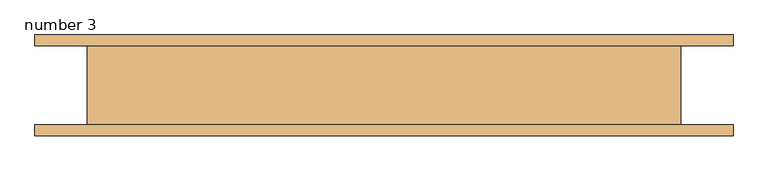
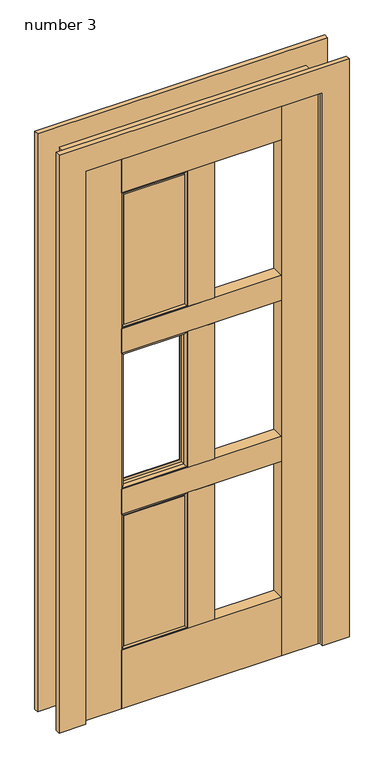
"""IFC4 building model written with IfcOpenShell, lengths in millimetres: door geometry, Door-Interior-Karona-K5660-6_Panel : number 3."""

from ifc_helpers import new_model, si_unit, frame, origin, origin_with_axes, place, context, project, spatial, polyline, ellipse_curve, outline, extrude, faceted_brep, source, transform, mapped, element, save
from ifc_brep_helpers import plane_surface, cylinder_surface, revolved_surface, advanced_brep


def number_3_9a47f452(model_context):
    return source(origin(), model_context, "Body", "SolidModel", [
        advanced_brep(
        [(-279.4, -15.2908, 1311.275), (-46.0375, -15.2908, 1311.275), (-57.3628137, -24.6126, 1299.9496863), (-268.0746863, -24.6126, 1299.9496863), (-57.1627, -46.3324899, 1300.1498), (-57.1627, -46.3324899, 820.7502), (-48.2727, -54.4576, 811.8602), (-48.2727, -54.4576, 1309.0398), (-268.2748, -46.3324899, 820.7502), (-268.2748, -46.3324899, 1300.1498), (-277.1648, -54.4576, 1309.0398), (-277.1648, -54.4576, 811.8602), (-46.0375, -54.4576, 809.625), (-279.4, -54.4576, 809.625), (-279.4, -15.2908, 809.625), (-46.0375, -15.2908, 809.625), (-57.1627, -34.7218, 820.7502), (-268.2748, -34.7218, 820.7502), (-47.3075, -24.6126, 1310.005), (-47.3075, -24.6126, 810.895), (-47.3075, -34.7218, 810.895), (-47.3075, -34.7218, 1310.005), (-278.13, -24.6126, 810.895), (-278.13, -24.6126, 1310.005), (-57.3628137, -24.6126, 820.9503137), (-268.0746863, -24.6126, 820.9503137), (-278.13, -34.7218, 810.895), (-279.4, -54.4576, 1311.275), (-268.2748, -34.7218, 1300.1498), (-278.13, -34.7218, 1310.005), (-46.0375, -54.4576, 1311.275), (-57.1627, -34.7218, 1300.1498)],
        [
            (0, 1),
            (1, 2, ellipse_curve(frame((-47.0685124, -25.5788135, 1310.2439876), z_axis=(-0.7071067811865475, 0.0, 0.7071067811865475), x_axis=(-0.7071067811865476, 0.0, -0.7071067811865474)), 14.6223259, 10.3395458)),
            (2, 3),
            (3, 0, ellipse_curve(frame((-278.3689876, -25.5788135, 1310.2439876), z_axis=(0.7071067811865475, 0.0, 0.7071067811865475), x_axis=(-0.7071067811865476, 0.0, 0.7071067811865474)), 14.6223259, 10.3395458)),
            (4, 5),
            (5, 6, ellipse_curve(frame((-48.2727, -45.531597, 811.8602), z_axis=(0.7071067811865475, 0.0, 0.7071067811865475), x_axis=(-0.7071067811865474, 0.0, 0.7071067811865476)), 12.6232745, 8.926003)),
            (6, 7),
            (7, 4, ellipse_curve(frame((-48.2727, -45.531597, 1309.0398), z_axis=(0.7071067811865475, 0.0, -0.7071067811865475), x_axis=(0.7071067811865474, 0.0, 0.7071067811865476)), 12.6232745, 8.926003)),
            (8, 9),
            (9, 10, ellipse_curve(frame((-277.1648, -45.531597, 1309.0398), z_axis=(-0.7071067811865475, 0.0, -0.7071067811865475), x_axis=(0.7071067811865474, 0.0, -0.7071067811865476)), 12.6232745, 8.926003)),
            (10, 11),
            (11, 8, ellipse_curve(frame((-277.1648, -45.531597, 811.8602), z_axis=(-0.7071067811865475, 0.0, 0.7071067811865475), x_axis=(-0.7071067811865474, 0.0, -0.7071067811865476)), 12.6232745, 8.926003)),
            (12, 13),
            (13, 14),
            (14, 15),
            (15, 12),
            (16, 17),
            (17, 8),
            (8, 5),
            (5, 16),
            (18, 19),
            (19, 20),
            (20, 21),
            (21, 18),
            (22, 19),
            (18, 23),
            (23, 22),
            (24, 25),
            (25, 3),
            (2, 24),
            (14, 25, ellipse_curve(frame((-278.3689876, -25.5788135, 810.6560124), z_axis=(0.7071067811865475, 0.0, -0.7071067811865475), x_axis=(0.7071067811865476, 0.0, 0.7071067811865474)), 14.6223259, 10.3395458)),
            (24, 15, ellipse_curve(frame((-47.0685124, -25.5788135, 810.6560124), z_axis=(-0.7071067811865475, 0.0, -0.7071067811865475), x_axis=(0.7071067811865476, 0.0, -0.7071067811865474)), 14.6223259, 10.3395458)),
            (22, 26),
            (26, 20),
            (13, 27),
            (27, 0),
            (0, 14),
            (17, 28),
            (28, 9),
            (23, 29),
            (29, 26),
            (27, 30),
            (30, 1),
            (28, 31),
            (31, 4),
            (4, 9),
            (21, 29),
            (30, 12),
            (15, 1),
            (31, 16),
            (6, 11),
            (10, 7),
        ],
        [
            cylinder_surface(frame((-279.4, -25.5788135, 1310.2439876), z_axis=(-1.0, 0.0, 0.0), x_axis=(0.0, 1.0, 0.0)), 10.3395458),
            cylinder_surface(frame((-48.2727, -45.531597, 1311.275), z_axis=(0.0, 0.0, 1.0), x_axis=(0.0, 1.0, 0.0)), 8.926003),
            cylinder_surface(frame((-277.1648, -45.531597, 809.625), z_axis=(0.0, 0.0, -1.0), x_axis=(0.0, 1.0, 0.0)), 8.926003),
            plane_surface(frame((-46.0375, -15.2908, 809.625), z_axis=(0.0, 0.0, -1.0), x_axis=(-1.0, 0.0, 0.0))),
            plane_surface(frame((-57.1627, -46.3324899, 820.7502), z_axis=(0.0, 0.0, 1.0), x_axis=(-1.0, 0.0, 0.0))),
            plane_surface(frame((-47.3075, -34.7218, 1310.005), z_axis=(-1.0, 0.0, 0.0), x_axis=(0.0, 0.0, -1.0))),
            plane_surface(frame((-47.3075, -24.6126, 1310.005), z_axis=(0.0, -1.0, 0.0), x_axis=(0.0, 0.0, -1.0))),
            cylinder_surface(frame((-46.0375, -25.5788135, 810.6560124), z_axis=(1.0, 0.0, 0.0), x_axis=(0.0, 1.0, 0.0)), 10.3395458),
            plane_surface(frame((-47.3075, -34.7218, 810.895), z_axis=(0.0, 0.0, 1.0), x_axis=(-1.0, 0.0, 0.0))),
            plane_surface(frame((-279.4, -15.2908, 809.625), z_axis=(-1.0, 0.0, 0.0), x_axis=(0.0, 0.0, 1.0))),
            plane_surface(frame((-268.2748, -46.3324899, 820.7502), z_axis=(1.0, 0.0, 0.0), x_axis=(0.0, 0.0, 1.0))),
            plane_surface(frame((-278.13, -34.7218, 810.895), z_axis=(1.0, 0.0, 0.0), x_axis=(0.0, 0.0, 1.0))),
            plane_surface(frame((-279.4, -15.2908, 1311.275), z_axis=(0.0, 0.0, 1.0), x_axis=(1.0, 0.0, 0.0))),
            plane_surface(frame((-268.2748, -46.3324899, 1300.1498), z_axis=(0.0, 0.0, -1.0), x_axis=(1.0, 0.0, 0.0))),
            plane_surface(frame((-278.13, -34.7218, 1310.005), z_axis=(0.0, 0.0, -1.0), x_axis=(1.0, 0.0, 0.0))),
            plane_surface(frame((-46.0375, -15.2908, 1311.275), z_axis=(1.0, 0.0, 0.0), x_axis=(0.0, 0.0, -1.0))),
            plane_surface(frame((-57.1627, -46.3324899, 1300.1498), z_axis=(-1.0, 0.0, 0.0), x_axis=(0.0, 0.0, -1.0))),
            plane_surface(frame((-57.1627, -34.7218, 1300.1498), z_axis=(0.0, 1.0, 0.0), x_axis=(0.0, 0.0, -1.0))),
            plane_surface(frame((-46.0375, -54.4576, 1311.275), z_axis=(0.0, -1.0, 0.0), x_axis=(0.0, 0.0, -1.0))),
            cylinder_surface(frame((-46.0375, -45.531597, 811.8602), z_axis=(1.0, 0.0, 0.0), x_axis=(0.0, 1.0, 0.0)), 8.926003),
            cylinder_surface(frame((-278.3689876, -25.5788135, 809.625), z_axis=(0.0, 0.0, -1.0), x_axis=(0.0, 1.0, 0.0)), 10.3395458),
            cylinder_surface(frame((-279.4, -45.531597, 1309.0398), z_axis=(-1.0, 0.0, 0.0), x_axis=(0.0, 1.0, 0.0)), 8.926003),
            cylinder_surface(frame((-47.0685124, -25.5788135, 1311.275), z_axis=(0.0, 0.0, 1.0), x_axis=(0.0, 1.0, 0.0)), 10.3395458),
        ],
        [
            (0, [[1, 2, 3, 4]]),
            (1, [[5, 6, 7, 8]]),
            (2, [[9, 10, 11, 12]]),
            (3, [[13, 14, 15, 16]]),
            (4, [[17, 18, 19, 20]]),
            (5, [[21, 22, 23, 24]]),
            (6, [[25, -21, 26, 27], [28, 29, -3, 30]]),
            (7, [[-15, 31, -28, 32]]),
            (8, [[-25, 33, 34, -22]]),
            (9, [[35, 36, 37, -14]]),
            (10, [[38, 39, -9, -18]]),
            (11, [[-27, 40, 41, -33]]),
            (12, [[42, 43, -1, -36]]),
            (13, [[44, 45, 46, -39]]),
            (14, [[-26, -24, 47, -40]]),
            (15, [[48, -16, 49, -43]]),
            (16, [[50, -20, -5, -45]]),
            (17, [[-34, -41, -47, -23], [-17, -50, -44, -38]]),
            (18, [[-13, -48, -42, -35], [51, -11, 52, -7]]),
            (19, [[-19, -12, -51, -6]]),
            (20, [[-37, -4, -29, -31]]),
            (21, [[-46, -8, -52, -10]]),
            (22, [[-49, -32, -30, -2]]),
        ],
    ),
        advanced_brep(
        [(-268.2748, -54.4576, 1893.8748), (-268.2748, -54.4576, 1414.4752), (-57.1627, -54.4576, 1414.4752), (-57.1627, -54.4576, 1893.8748), (-268.2748, -34.7218, 1893.8748), (-268.2748, -36.0454899, 1893.8748), (-57.1627, -36.0454899, 1893.8748), (-57.1627, -34.7218, 1893.8748), (-57.1627, -44.5515929, 1893.8748), (-268.2748, -44.5515929, 1893.8748), (-57.1627, -34.7218, 1414.4752), (-57.1627, -36.0454899, 1414.4752), (-268.2748, -36.0454899, 1414.4752), (-268.2748, -34.7218, 1414.4752), (-268.2748, -44.5515929, 1414.4752), (-57.1627, -44.5515929, 1414.4752), (-87.1686653, -44.5515929, 1863.8688347), (-238.2688347, -44.5515929, 1863.8688347), (-87.1686653, -44.5515929, 1444.4811653), (-238.2688347, -44.5515929, 1444.4811653)],
        [
            (0, 1),
            (1, 2),
            (2, 3),
            (3, 0),
            (4, 5),
            (5, 6),
            (6, 7),
            (7, 4),
            (3, 8),
            (8, 9),
            (9, 0),
            (10, 11),
            (11, 12),
            (12, 13),
            (13, 10),
            (1, 14),
            (14, 15),
            (15, 2),
            (9, 14),
            (12, 5),
            (4, 13),
            (6, 11),
            (10, 7),
            (15, 8),
            (16, 6, ellipse_curve(frame((-55.2243315, -100.0605261, 1895.8131685), z_axis=(0.7071067811865475, 0.0, -0.7071067811865475), x_axis=(-0.7071067811865476, 0.0, -0.7071067811865474)), 90.5724254, 64.0443762)),
            (5, 17, ellipse_curve(frame((-270.2131685, -100.0605261, 1895.8131685), z_axis=(-0.7071067811865475, 0.0, -0.7071067811865475), x_axis=(-0.7071067811865476, 0.0, 0.7071067811865474)), 90.5724254, 64.0443762)),
            (17, 16),
            (18, 11, ellipse_curve(frame((-55.2243315, -100.0605261, 1412.5368315), z_axis=(-0.7071067811865475, 0.0, -0.7071067811865475), x_axis=(-0.7071067811865474, 0.0, 0.7071067811865476)), 90.5724254, 64.0443762)),
            (16, 18),
            (19, 12, ellipse_curve(frame((-270.2131685, -100.0605261, 1412.5368315), z_axis=(-0.7071067811865475, 0.0, 0.7071067811865475), x_axis=(0.7071067811865476, 0.0, 0.7071067811865474)), 90.5724254, 64.0443762)),
            (18, 19),
            (19, 17),
        ],
        [
            plane_surface(frame((-57.1627, -54.4576, 1893.8748), z_axis=(0.0, -1.0, 0.0), x_axis=(0.0, 0.0, -1.0))),
            plane_surface(frame((-57.1627, -34.7218, 1893.8748), z_axis=(0.0, 0.0, 1.0), x_axis=(1.0, 0.0, 0.0))),
            plane_surface(frame((-57.1627, -34.7218, 1414.4752), z_axis=(0.0, 0.0, -1.0), x_axis=(-1.0, 0.0, 0.0))),
            plane_surface(frame((-268.2748, -54.4576, 1893.8748), z_axis=(-1.0, 0.0, 0.0), x_axis=(0.0, 0.0, -1.0))),
            plane_surface(frame((-57.1627, -34.7218, 1893.8748), z_axis=(1.0, 0.0, 0.0), x_axis=(0.0, 0.0, -1.0))),
            plane_surface(frame((-268.2748, -34.7218, 1893.8748), z_axis=(0.0, 1.0, 0.0), x_axis=(0.0, 0.0, -1.0))),
            revolved_surface(polyline([(-334.2575446888527, -100.0605261, 1831.7687923), (8.820044688852704, -100.0605261, 1831.7687923)]), (-279.4, -100.0605261, 1895.8131685), (-1.0, 0.0, 0.0)),
            revolved_surface(polyline([(-119.2687077, -100.0605261, 1959.8575446888528), (-119.2687077, -100.0605261, 1348.4924553111473)]), (-55.2243315, -100.0605261, 1905.0), (0.0, 0.0, 1.0)),
            revolved_surface(polyline([(8.820044688852683, -100.0605261, 1476.5812077), (-334.2575446888527, -100.0605261, 1476.5812077)]), (-46.0375, -100.0605261, 1412.5368315), (1.0, 0.0, 0.0)),
            revolved_surface(polyline([(-206.1687923, -100.0605261, 1348.4924553111473), (-206.1687923, -100.0605261, 1959.8575446888526)]), (-270.2131685, -100.0605261, 1403.35), (0.0, 0.0, -1.0)),
            plane_surface(frame((-279.4, -44.5515929, 1403.35), z_axis=(0.0, 1.0, 0.0), x_axis=(0.0, 0.0, 1.0))),
        ],
        [
            (0, [[1, 2, 3, 4]]),
            (1, [[5, 6, 7, 8]]),
            (1, [[9, 10, 11, -4]]),
            (2, [[12, 13, 14, 15]]),
            (2, [[16, 17, 18, -2]]),
            (3, [[-11, 19, -16, -1]]),
            (3, [[-14, 20, -5, 21]]),
            (4, [[-7, 22, -12, 23]]),
            (4, [[-18, 24, -9, -3]]),
            (5, [[-23, -15, -21, -8]]),
            (6, [[25, -6, 26, 27]]),
            (7, [[28, -22, -25, 29]]),
            (8, [[30, -13, -28, 31]]),
            (9, [[-26, -20, -30, 32]]),
            (10, [[-24, -17, -19, -10], [-32, -31, -29, -27]]),
        ],
    ),
        advanced_brep(
        [(-268.2748, -24.6126, 1893.8748), (-268.2748, -24.6126, 1414.4752), (-57.1627, -24.6126, 1414.4752), (-57.1627, -24.6126, 1893.8748), (-239.4448579, -15.4432, 1443.3051421), (-239.4448579, -15.4432, 1865.0448579), (-85.9926421, -15.4432, 1865.0448579), (-85.9926421, -15.4432, 1443.3051421), (-57.1627, -23.2889101, 1893.8748), (-268.2748, -23.2889101, 1893.8748), (-268.2748, -23.2889101, 1414.4752), (-57.1627, -23.2889101, 1414.4752)],
        [
            (0, 1),
            (1, 2),
            (2, 3),
            (3, 0),
            (4, 5),
            (5, 6),
            (6, 7),
            (7, 4),
            (3, 8),
            (8, 9),
            (9, 0),
            (1, 10),
            (10, 11),
            (11, 2),
            (7, 11, ellipse_curve(frame((-55.2243315, 40.7261261, 1412.5368315), z_axis=(0.7071067811865475, 0.0, 0.7071067811865475), x_axis=(0.7071067811865476, 0.0, -0.7071067811865474)), 90.5724254, 64.0443762)),
            (10, 4, ellipse_curve(frame((-270.2131685, 40.7261261, 1412.5368315), z_axis=(-0.7071067811865475, 0.0, 0.7071067811865475), x_axis=(0.7071067811865476, 0.0, 0.7071067811865474)), 90.5724254, 64.0443762)),
            (10, 9),
            (9, 5, ellipse_curve(frame((-270.2131685, 40.7261261, 1895.8131685), z_axis=(0.7071067811865475, 0.0, 0.7071067811865475), x_axis=(0.7071067811865474, 0.0, -0.7071067811865476)), 90.5724254, 64.0443762)),
            (8, 6, ellipse_curve(frame((-55.2243315, 40.7261261, 1895.8131685), z_axis=(0.7071067811865475, 0.0, -0.7071067811865475), x_axis=(-0.7071067811865476, 0.0, -0.7071067811865474)), 90.5724254, 64.0443762)),
            (8, 11),
        ],
        [
            plane_surface(frame((-57.1627, -24.6126, 1893.8748), z_axis=(0.0, -1.0, 0.0), x_axis=(0.0, 0.0, -1.0))),
            plane_surface(frame((-268.2748, -15.4432, 1893.8748), z_axis=(0.0, 1.0, 0.0), x_axis=(0.0, 0.0, -1.0))),
            plane_surface(frame((-57.1627, -34.7218, 1893.8748), z_axis=(0.0, 0.0, 1.0), x_axis=(1.0, 0.0, 0.0))),
            plane_surface(frame((-57.1627, -34.7218, 1414.4752), z_axis=(0.0, 0.0, -1.0), x_axis=(-1.0, 0.0, 0.0))),
            revolved_surface(polyline([(8.820044688852711, 40.7261261, 1476.5812077), (-334.2575446888527, 40.7261261, 1476.5812077)]), (-46.0375, 40.7261261, 1412.5368315), (1.0, 0.0, 0.0)),
            revolved_surface(polyline([(-206.1687923, 40.7261261, 1348.4924553111473), (-206.1687923, 40.7261261, 1959.8575446888528)]), (-270.2131685, 40.7261261, 1403.35), (0.0, 0.0, -1.0)),
            revolved_surface(polyline([(-334.2575446888527, 40.7261261, 1831.7687923), (8.820044688852704, 40.7261261, 1831.7687923)]), (-279.4, 40.7261261, 1895.8131685), (-1.0, 0.0, 0.0)),
            revolved_surface(polyline([(-119.2687077, 40.7261261, 1959.8575446888528), (-119.2687077, 40.7261261, 1348.4924553111473)]), (-55.2243315, 40.7261261, 1905.0), (0.0, 0.0, 1.0)),
            plane_surface(frame((-268.2748, -24.6126, 1893.8748), z_axis=(-1.0, 0.0, 0.0), x_axis=(0.0, 0.0, -1.0))),
            plane_surface(frame((-57.1627, -15.4432, 1893.8748), z_axis=(1.0, 0.0, 0.0), x_axis=(0.0, 0.0, -1.0))),
        ],
        [
            (0, [[1, 2, 3, 4]]),
            (1, [[5, 6, 7, 8]]),
            (2, [[9, 10, 11, -4]]),
            (3, [[12, 13, 14, -2]]),
            (4, [[-8, 15, -13, 16]]),
            (5, [[17, 18, -5, -16]]),
            (6, [[-10, 19, -6, -18]]),
            (7, [[20, -15, -7, -19]]),
            (8, [[-11, -17, -12, -1]]),
            (9, [[-14, -20, -9, -3]]),
        ],
    ),
        advanced_brep(
        [(-279.4, -15.2908, 1905.0), (-46.0375, -15.2908, 1905.0), (-57.3628137, -24.6126, 1893.6746863), (-268.0746863, -24.6126, 1893.6746863), (-57.1627, -46.3324899, 1893.8748), (-57.1627, -46.3324899, 1414.4752), (-48.2727, -54.4576, 1405.5852), (-48.2727, -54.4576, 1902.7648), (-268.2748, -46.3324899, 1414.4752), (-268.2748, -46.3324899, 1893.8748), (-277.1648, -54.4576, 1902.7648), (-277.1648, -54.4576, 1405.5852), (-46.0375, -54.4576, 1403.35), (-279.4, -54.4576, 1403.35), (-279.4, -15.2908, 1403.35), (-46.0375, -15.2908, 1403.35), (-57.1627, -34.7218, 1414.4752), (-268.2748, -34.7218, 1414.4752), (-47.3075, -24.6126, 1903.73), (-47.3075, -24.6126, 1404.62), (-47.3075, -34.7218, 1404.62), (-47.3075, -34.7218, 1903.73), (-278.13, -24.6126, 1404.62), (-278.13, -24.6126, 1903.73), (-57.3628137, -24.6126, 1414.6753137), (-268.0746863, -24.6126, 1414.6753137), (-278.13, -34.7218, 1404.62), (-279.4, -54.4576, 1905.0), (-268.2748, -34.7218, 1893.8748), (-278.13, -34.7218, 1903.73), (-46.0375, -54.4576, 1905.0), (-57.1627, -34.7218, 1893.8748)],
        [
            (0, 1),
            (1, 2, ellipse_curve(frame((-47.0685124, -25.5788135, 1903.9689876), z_axis=(-0.7071067811865475, 0.0, 0.7071067811865475), x_axis=(-0.7071067811865476, 0.0, -0.7071067811865474)), 14.6223259, 10.3395458)),
            (2, 3),
            (3, 0, ellipse_curve(frame((-278.3689876, -25.5788135, 1903.9689876), z_axis=(0.7071067811865475, 0.0, 0.7071067811865475), x_axis=(-0.7071067811865476, 0.0, 0.7071067811865474)), 14.6223259, 10.3395458)),
            (4, 5),
            (5, 6, ellipse_curve(frame((-48.2727, -45.531597, 1405.5852), z_axis=(0.7071067811865475, 0.0, 0.7071067811865475), x_axis=(-0.7071067811865474, 0.0, 0.7071067811865476)), 12.6232745, 8.926003)),
            (6, 7),
            (7, 4, ellipse_curve(frame((-48.2727, -45.531597, 1902.7648), z_axis=(0.7071067811865475, 0.0, -0.7071067811865475), x_axis=(0.7071067811865474, 0.0, 0.7071067811865476)), 12.6232745, 8.926003)),
            (8, 9),
            (9, 10, ellipse_curve(frame((-277.1648, -45.531597, 1902.7648), z_axis=(-0.7071067811865475, 0.0, -0.7071067811865475), x_axis=(0.7071067811865474, 0.0, -0.7071067811865476)), 12.6232745, 8.926003)),
            (10, 11),
            (11, 8, ellipse_curve(frame((-277.1648, -45.531597, 1405.5852), z_axis=(-0.7071067811865475, 0.0, 0.7071067811865475), x_axis=(-0.7071067811865474, 0.0, -0.7071067811865476)), 12.6232745, 8.926003)),
            (12, 13),
            (13, 14),
            (14, 15),
            (15, 12),
            (16, 17),
            (17, 8),
            (8, 5),
            (5, 16),
            (18, 19),
            (19, 20),
            (20, 21),
            (21, 18),
            (22, 19),
            (18, 23),
            (23, 22),
            (24, 25),
            (25, 3),
            (2, 24),
            (14, 25, ellipse_curve(frame((-278.3689876, -25.5788135, 1404.3810124), z_axis=(0.7071067811865475, 0.0, -0.7071067811865475), x_axis=(0.7071067811865476, 0.0, 0.7071067811865474)), 14.6223259, 10.3395458)),
            (24, 15, ellipse_curve(frame((-47.0685124, -25.5788135, 1404.3810124), z_axis=(-0.7071067811865475, 0.0, -0.7071067811865475), x_axis=(0.7071067811865476, 0.0, -0.7071067811865474)), 14.6223259, 10.3395458)),
            (22, 26),
            (26, 20),
            (13, 27),
            (27, 0),
            (0, 14),
            (17, 28),
            (28, 9),
            (23, 29),
            (29, 26),
            (27, 30),
            (30, 1),
            (28, 31),
            (31, 4),
            (4, 9),
            (21, 29),
            (30, 12),
            (15, 1),
            (31, 16),
            (6, 11),
            (10, 7),
        ],
        [
            cylinder_surface(frame((-279.4, -25.5788135, 1903.9689876), z_axis=(-1.0, 0.0, 0.0), x_axis=(0.0, 1.0, 0.0)), 10.3395458),
            cylinder_surface(frame((-48.2727, -45.531597, 1905.0), z_axis=(0.0, 0.0, 1.0), x_axis=(0.0, 1.0, 0.0)), 8.926003),
            cylinder_surface(frame((-277.1648, -45.531597, 1403.35), z_axis=(0.0, 0.0, -1.0), x_axis=(0.0, 1.0, 0.0)), 8.926003),
            plane_surface(frame((-46.0375, -15.2908, 1403.35), z_axis=(0.0, 0.0, -1.0), x_axis=(-1.0, 0.0, 0.0))),
            plane_surface(frame((-57.1627, -46.3324899, 1414.4752), z_axis=(0.0, 0.0, 1.0), x_axis=(-1.0, 0.0, 0.0))),
            plane_surface(frame((-47.3075, -34.7218, 1903.73), z_axis=(-1.0, 0.0, 0.0), x_axis=(0.0, 0.0, -1.0))),
            plane_surface(frame((-47.3075, -24.6126, 1903.73), z_axis=(0.0, -1.0, 0.0), x_axis=(0.0, 0.0, -1.0))),
            cylinder_surface(frame((-46.0375, -25.5788135, 1404.3810124), z_axis=(1.0, 0.0, 0.0), x_axis=(0.0, 1.0, 0.0)), 10.3395458),
            plane_surface(frame((-47.3075, -34.7218, 1404.62), z_axis=(0.0, 0.0, 1.0), x_axis=(-1.0, 0.0, 0.0))),
            plane_surface(frame((-279.4, -15.2908, 1403.35), z_axis=(-1.0, 0.0, 0.0), x_axis=(0.0, 0.0, 1.0))),
            plane_surface(frame((-268.2748, -46.3324899, 1414.4752), z_axis=(1.0, 0.0, 0.0), x_axis=(0.0, 0.0, 1.0))),
            plane_surface(frame((-278.13, -34.7218, 1404.62), z_axis=(1.0, 0.0, 0.0), x_axis=(0.0, 0.0, 1.0))),
            plane_surface(frame((-279.4, -15.2908, 1905.0), z_axis=(0.0, 0.0, 1.0), x_axis=(1.0, 0.0, 0.0))),
            plane_surface(frame((-268.2748, -46.3324899, 1893.8748), z_axis=(0.0, 0.0, -1.0), x_axis=(1.0, 0.0, 0.0))),
            plane_surface(frame((-278.13, -34.7218, 1903.73), z_axis=(0.0, 0.0, -1.0), x_axis=(1.0, 0.0, 0.0))),
            plane_surface(frame((-46.0375, -15.2908, 1905.0), z_axis=(1.0, 0.0, 0.0), x_axis=(0.0, 0.0, -1.0))),
            plane_surface(frame((-57.1627, -46.3324899, 1893.8748), z_axis=(-1.0, 0.0, 0.0), x_axis=(0.0, 0.0, -1.0))),
            plane_surface(frame((-57.1627, -34.7218, 1893.8748), z_axis=(0.0, 1.0, 0.0), x_axis=(0.0, 0.0, -1.0))),
            plane_surface(frame((-46.0375, -54.4576, 1905.0), z_axis=(0.0, -1.0, 0.0), x_axis=(0.0, 0.0, -1.0))),
            cylinder_surface(frame((-46.0375, -45.531597, 1405.5852), z_axis=(1.0, 0.0, 0.0), x_axis=(0.0, 1.0, 0.0)), 8.926003),
            cylinder_surface(frame((-278.3689876, -25.5788135, 1403.35), z_axis=(0.0, 0.0, -1.0), x_axis=(0.0, 1.0, 0.0)), 10.3395458),
            cylinder_surface(frame((-279.4, -45.531597, 1902.7648), z_axis=(-1.0, 0.0, 0.0), x_axis=(0.0, 1.0, 0.0)), 8.926003),
            cylinder_surface(frame((-47.0685124, -25.5788135, 1905.0), z_axis=(0.0, 0.0, 1.0), x_axis=(0.0, 1.0, 0.0)), 10.3395458),
        ],
        [
            (0, [[1, 2, 3, 4]]),
            (1, [[5, 6, 7, 8]]),
            (2, [[9, 10, 11, 12]]),
            (3, [[13, 14, 15, 16]]),
            (4, [[17, 18, 19, 20]]),
            (5, [[21, 22, 23, 24]]),
            (6, [[25, -21, 26, 27], [28, 29, -3, 30]]),
            (7, [[-15, 31, -28, 32]]),
            (8, [[-25, 33, 34, -22]]),
            (9, [[35, 36, 37, -14]]),
            (10, [[38, 39, -9, -18]]),
            (11, [[-27, 40, 41, -33]]),
            (12, [[42, 43, -1, -36]]),
            (13, [[44, 45, 46, -39]]),
            (14, [[-26, -24, 47, -40]]),
            (15, [[48, -16, 49, -43]]),
            (16, [[50, -20, -5, -45]]),
            (17, [[-34, -41, -47, -23], [-17, -50, -44, -38]]),
            (18, [[-13, -48, -42, -35], [51, -11, 52, -7]]),
            (19, [[-19, -12, -51, -6]]),
            (20, [[-37, -4, -29, -31]]),
            (21, [[-46, -8, -52, -10]]),
            (22, [[-49, -32, -30, -2]]),
        ],
    ),
        advanced_brep(
        [(-268.2748, -34.7218, 706.4248), (-268.2748, -36.0454899, 706.4248), (-57.1627, -36.0454899, 706.4248), (-57.1627, -34.7218, 706.4248), (-57.1627, -54.4576, 706.4248), (-57.1627, -44.5515929, 706.4248), (-268.2748, -44.5515929, 706.4248), (-268.2748, -54.4576, 706.4248), (-57.1627, -34.7218, 227.0252), (-57.1627, -36.0454899, 227.0252), (-268.2748, -36.0454899, 227.0252), (-268.2748, -34.7218, 227.0252), (-268.2748, -54.4576, 227.0252), (-268.2748, -44.5515929, 227.0252), (-57.1627, -44.5515929, 227.0252), (-57.1627, -54.4576, 227.0252), (-87.1686653, -44.5515929, 676.4188347), (-238.2688347, -44.5515929, 676.4188347), (-87.1686653, -44.5515929, 257.0311653), (-238.2688347, -44.5515929, 257.0311653)],
        [
            (0, 1),
            (1, 2),
            (2, 3),
            (3, 0),
            (4, 5),
            (5, 6),
            (6, 7),
            (7, 4),
            (8, 9),
            (9, 10),
            (10, 11),
            (11, 8),
            (12, 13),
            (13, 14),
            (14, 15),
            (15, 12),
            (6, 13),
            (12, 7),
            (10, 1),
            (0, 11),
            (15, 4),
            (2, 9),
            (8, 3),
            (14, 5),
            (16, 2, ellipse_curve(frame((-55.2243315, -100.0605261, 708.3631685), z_axis=(0.7071067811865475, 0.0, -0.7071067811865475), x_axis=(-0.7071067811865476, 0.0, -0.7071067811865474)), 90.5724254, 64.0443762)),
            (1, 17, ellipse_curve(frame((-270.2131685, -100.0605261, 708.3631685), z_axis=(-0.7071067811865475, 0.0, -0.7071067811865475), x_axis=(-0.7071067811865476, 0.0, 0.7071067811865474)), 90.5724254, 64.0443762)),
            (17, 16),
            (18, 9, ellipse_curve(frame((-55.2243315, -100.0605261, 225.0868315), z_axis=(-0.7071067811865475, 0.0, -0.7071067811865475), x_axis=(-0.7071067811865474, 0.0, 0.7071067811865476)), 90.5724254, 64.0443762)),
            (16, 18),
            (19, 10, ellipse_curve(frame((-270.2131685, -100.0605261, 225.0868315), z_axis=(-0.7071067811865475, 0.0, 0.7071067811865475), x_axis=(0.7071067811865476, 0.0, 0.7071067811865474)), 90.5724254, 64.0443762)),
            (18, 19),
            (19, 17),
        ],
        [
            plane_surface(frame((-57.1627, -34.7218, 706.4248), z_axis=(0.0, 0.0, 1.0), x_axis=(1.0, 0.0, 0.0))),
            plane_surface(frame((-57.1627, -34.7218, 227.0252), z_axis=(0.0, 0.0, -1.0), x_axis=(-1.0, 0.0, 0.0))),
            plane_surface(frame((-268.2748, -54.4576, 706.4248), z_axis=(-1.0, 0.0, 0.0), x_axis=(0.0, 0.0, -1.0))),
            plane_surface(frame((-57.1627, -54.4576, 706.4248), z_axis=(0.0, -1.0, 0.0), x_axis=(0.0, 0.0, -1.0))),
            plane_surface(frame((-57.1627, -34.7218, 706.4248), z_axis=(1.0, 0.0, 0.0), x_axis=(0.0, 0.0, -1.0))),
            plane_surface(frame((-268.2748, -34.7218, 706.4248), z_axis=(0.0, 1.0, 0.0), x_axis=(0.0, 0.0, -1.0))),
            revolved_surface(polyline([(-334.2575446888527, -100.0605261, 644.3187923), (8.820044688852704, -100.0605261, 644.3187923)]), (-279.4, -100.0605261, 708.3631685), (-1.0, 0.0, 0.0)),
            revolved_surface(polyline([(-119.2687077, -100.0605261, 772.4075446888527), (-119.2687077, -100.0605261, 161.04245531114725)]), (-55.2243315, -100.0605261, 717.55), (0.0, 0.0, 1.0)),
            revolved_surface(polyline([(8.820044688852683, -100.0605261, 289.1312077), (-334.2575446888527, -100.0605261, 289.1312077)]), (-46.0375, -100.0605261, 225.0868315), (1.0, 0.0, 0.0)),
            revolved_surface(polyline([(-206.1687923, -100.0605261, 161.0424553111473), (-206.1687923, -100.0605261, 772.4075446888527)]), (-270.2131685, -100.0605261, 215.9), (0.0, 0.0, -1.0)),
            plane_surface(frame((-279.4, -44.5515929, 215.9), z_axis=(0.0, 1.0, 0.0), x_axis=(0.0, 0.0, 1.0))),
        ],
        [
            (0, [[1, 2, 3, 4]]),
            (0, [[5, 6, 7, 8]]),
            (1, [[9, 10, 11, 12]]),
            (1, [[13, 14, 15, 16]]),
            (2, [[-7, 17, -13, 18]]),
            (2, [[-11, 19, -1, 20]]),
            (3, [[-18, -16, 21, -8]]),
            (4, [[-3, 22, -9, 23]]),
            (4, [[-15, 24, -5, -21]]),
            (5, [[-23, -12, -20, -4]]),
            (6, [[25, -2, 26, 27]]),
            (7, [[28, -22, -25, 29]]),
            (8, [[30, -10, -28, 31]]),
            (9, [[-26, -19, -30, 32]]),
            (10, [[-24, -14, -17, -6], [-32, -31, -29, -27]]),
        ],
    ),
        advanced_brep(
        [(-57.1627, -24.6126, 706.4248), (-57.1627, -23.2889101, 706.4248), (-268.2748, -23.2889101, 706.4248), (-268.2748, -24.6126, 706.4248), (-268.2748, -24.6126, 227.0252), (-268.2748, -23.2889101, 227.0252), (-57.1627, -23.2889101, 227.0252), (-57.1627, -24.6126, 227.0252), (-239.4448579, -15.4432, 255.8551421), (-239.4448579, -15.4432, 677.5948579), (-85.9926421, -15.4432, 677.5948579), (-85.9926421, -15.4432, 255.8551421)],
        [
            (0, 1),
            (1, 2),
            (2, 3),
            (3, 0),
            (4, 5),
            (5, 6),
            (6, 7),
            (7, 4),
            (3, 4),
            (7, 0),
            (8, 9),
            (9, 10),
            (10, 11),
            (11, 8),
            (11, 6, ellipse_curve(frame((-55.2243315, 40.7261261, 225.0868315), z_axis=(0.7071067811865475, 0.0, 0.7071067811865475), x_axis=(0.7071067811865476, 0.0, -0.7071067811865474)), 90.5724254, 64.0443762)),
            (5, 8, ellipse_curve(frame((-270.2131685, 40.7261261, 225.0868315), z_axis=(-0.7071067811865475, 0.0, 0.7071067811865475), x_axis=(0.7071067811865476, 0.0, 0.7071067811865474)), 90.5724254, 64.0443762)),
            (5, 2),
            (2, 9, ellipse_curve(frame((-270.2131685, 40.7261261, 708.3631685), z_axis=(0.7071067811865475, 0.0, 0.7071067811865475), x_axis=(0.7071067811865474, 0.0, -0.7071067811865476)), 90.5724254, 64.0443762)),
            (1, 10, ellipse_curve(frame((-55.2243315, 40.7261261, 708.3631685), z_axis=(0.7071067811865475, 0.0, -0.7071067811865475), x_axis=(-0.7071067811865476, 0.0, -0.7071067811865474)), 90.5724254, 64.0443762)),
            (1, 6),
        ],
        [
            plane_surface(frame((-57.1627, -34.7218, 706.4248), z_axis=(0.0, 0.0, 1.0), x_axis=(1.0, 0.0, 0.0))),
            plane_surface(frame((-57.1627, -34.7218, 227.0252), z_axis=(0.0, 0.0, -1.0), x_axis=(-1.0, 0.0, 0.0))),
            plane_surface(frame((-57.1627, -24.6126, 706.4248), z_axis=(0.0, -1.0, 0.0), x_axis=(0.0, 0.0, -1.0))),
            plane_surface(frame((-268.2748, -15.4432, 706.4248), z_axis=(0.0, 1.0, 0.0), x_axis=(0.0, 0.0, -1.0))),
            revolved_surface(polyline([(8.820044688852711, 40.7261261, 289.1312077), (-334.2575446888527, 40.7261261, 289.1312077)]), (-46.0375, 40.7261261, 225.0868315), (1.0, 0.0, 0.0)),
            revolved_surface(polyline([(-206.1687923, 40.7261261, 161.0424553111473), (-206.1687923, 40.7261261, 772.4075446888527)]), (-270.2131685, 40.7261261, 215.9), (0.0, 0.0, -1.0)),
            revolved_surface(polyline([(-334.2575446888527, 40.7261261, 644.3187923), (8.820044688852704, 40.7261261, 644.3187923)]), (-279.4, 40.7261261, 708.3631685), (-1.0, 0.0, 0.0)),
            revolved_surface(polyline([(-119.2687077, 40.7261261, 772.4075446888527), (-119.2687077, 40.7261261, 161.04245531114736)]), (-55.2243315, 40.7261261, 717.55), (0.0, 0.0, 1.0)),
            plane_surface(frame((-268.2748, -24.6126, 706.4248), z_axis=(-1.0, 0.0, 0.0), x_axis=(0.0, 0.0, -1.0))),
            plane_surface(frame((-57.1627, -15.4432, 706.4248), z_axis=(1.0, 0.0, 0.0), x_axis=(0.0, 0.0, -1.0))),
        ],
        [
            (0, [[1, 2, 3, 4]]),
            (1, [[5, 6, 7, 8]]),
            (2, [[9, -8, 10, -4]]),
            (3, [[11, 12, 13, 14]]),
            (4, [[-14, 15, -6, 16]]),
            (5, [[17, 18, -11, -16]]),
            (6, [[-2, 19, -12, -18]]),
            (7, [[20, -15, -13, -19]]),
            (8, [[-3, -17, -5, -9]]),
            (9, [[-7, -20, -1, -10]]),
        ],
    ),
        advanced_brep(
        [(-279.4, -15.2908, 717.55), (-46.0375, -15.2908, 717.55), (-57.3628137, -24.6126, 706.2246863), (-268.0746863, -24.6126, 706.2246863), (-57.1627, -46.3324899, 706.4248), (-57.1627, -46.3324899, 227.0252), (-48.2727, -54.4576, 218.1352), (-48.2727, -54.4576, 715.3148), (-279.4, -54.4576, 215.9), (-46.0375, -54.4576, 215.9), (-46.0375, -54.4576, 717.55), (-279.4, -54.4576, 717.55), (-277.1648, -54.4576, 218.1352), (-277.1648, -54.4576, 715.3148), (-279.4, -15.2908, 215.9), (-46.0375, -15.2908, 215.9), (-57.1627, -34.7218, 227.0252), (-268.2748, -34.7218, 227.0252), (-268.2748, -46.3324899, 227.0252), (-47.3075, -24.6126, 217.17), (-278.13, -24.6126, 217.17), (-278.13, -34.7218, 217.17), (-47.3075, -34.7218, 217.17), (-268.2748, -34.7218, 706.4248), (-268.2748, -46.3324899, 706.4248), (-278.13, -24.6126, 716.28), (-278.13, -34.7218, 716.28), (-57.1627, -34.7218, 706.4248), (-47.3075, -24.6126, 716.28), (-47.3075, -34.7218, 716.28), (-57.3628137, -24.6126, 227.2253137), (-268.0746863, -24.6126, 227.2253137)],
        [
            (0, 1),
            (1, 2, ellipse_curve(frame((-47.0685124, -25.5788135, 716.5189876), z_axis=(-0.7071067811865475, 0.0, 0.7071067811865475), x_axis=(-0.7071067811865476, 0.0, -0.7071067811865474)), 14.6223259, 10.3395458)),
            (2, 3),
            (3, 0, ellipse_curve(frame((-278.3689876, -25.5788135, 716.5189876), z_axis=(0.7071067811865475, 0.0, 0.7071067811865475), x_axis=(-0.7071067811865476, 0.0, 0.7071067811865474)), 14.6223259, 10.3395458)),
            (4, 5),
            (5, 6, ellipse_curve(frame((-48.2727, -45.531597, 218.1352), z_axis=(0.7071067811865475, 0.0, 0.7071067811865475), x_axis=(-0.7071067811865474, 0.0, 0.7071067811865476)), 12.6232745, 8.926003)),
            (6, 7),
            (7, 4, ellipse_curve(frame((-48.2727, -45.531597, 715.3148), z_axis=(0.7071067811865475, 0.0, -0.7071067811865475), x_axis=(0.7071067811865474, 0.0, 0.7071067811865476)), 12.6232745, 8.926003)),
            (8, 9),
            (9, 10),
            (10, 11),
            (11, 8),
            (6, 12),
            (12, 13),
            (13, 7),
            (8, 14),
            (14, 15),
            (15, 9),
            (16, 17),
            (17, 18),
            (18, 5),
            (5, 16),
            (19, 20),
            (20, 21),
            (21, 22),
            (22, 19),
            (11, 0),
            (0, 14),
            (17, 23),
            (23, 24),
            (24, 18),
            (20, 25),
            (25, 26),
            (26, 21),
            (10, 1),
            (23, 27),
            (27, 4),
            (4, 24),
            (25, 28),
            (28, 29),
            (29, 26),
            (15, 1),
            (27, 16),
            (29, 22),
            (28, 19),
            (30, 31),
            (31, 3),
            (2, 30),
            (15, 30, ellipse_curve(frame((-47.0685124, -25.5788135, 216.9310124), z_axis=(0.7071067811865475, 0.0, 0.7071067811865475), x_axis=(-0.7071067811865474, 0.0, 0.7071067811865476)), 14.6223259, 10.3395458)),
            (24, 13, ellipse_curve(frame((-277.1648, -45.531597, 715.3148), z_axis=(-0.7071067811865475, 0.0, -0.7071067811865475), x_axis=(0.7071067811865474, 0.0, -0.7071067811865476)), 12.6232745, 8.926003)),
            (12, 18, ellipse_curve(frame((-277.1648, -45.531597, 218.1352), z_axis=(-0.7071067811865475, 0.0, 0.7071067811865475), x_axis=(-0.7071067811865474, 0.0, -0.7071067811865476)), 12.6232745, 8.926003)),
            (14, 31, ellipse_curve(frame((-278.3689876, -25.5788135, 216.9310124), z_axis=(0.7071067811865475, 0.0, -0.7071067811865475), x_axis=(0.7071067811865476, 0.0, 0.7071067811865474)), 14.6223259, 10.3395458)),
        ],
        [
            cylinder_surface(frame((-279.4, -25.5788135, 716.5189876), z_axis=(-1.0, 0.0, 0.0), x_axis=(0.0, 1.0, 0.0)), 10.3395458),
            cylinder_surface(frame((-48.2727, -45.531597, 717.55), z_axis=(0.0, 0.0, 1.0), x_axis=(0.0, 1.0, 0.0)), 8.926003),
            plane_surface(frame((-46.0375, -54.4576, 717.55), z_axis=(0.0, -1.0, 0.0), x_axis=(0.0, 0.0, -1.0))),
            plane_surface(frame((-46.0375, -15.2908, 215.9), z_axis=(0.0, 0.0, -1.0), x_axis=(-1.0, 0.0, 0.0))),
            plane_surface(frame((-57.1627, -46.3324899, 227.0252), z_axis=(0.0, 0.0, 1.0), x_axis=(-1.0, 0.0, 0.0))),
            plane_surface(frame((-47.3075, -34.7218, 217.17), z_axis=(0.0, 0.0, 1.0), x_axis=(-1.0, 0.0, 0.0))),
            plane_surface(frame((-279.4, -15.2908, 215.9), z_axis=(-1.0, 0.0, 0.0), x_axis=(0.0, 0.0, 1.0))),
            plane_surface(frame((-268.2748, -46.3324899, 227.0252), z_axis=(1.0, 0.0, 0.0), x_axis=(0.0, 0.0, 1.0))),
            plane_surface(frame((-278.13, -34.7218, 217.17), z_axis=(1.0, 0.0, 0.0), x_axis=(0.0, 0.0, 1.0))),
            plane_surface(frame((-279.4, -15.2908, 717.55), z_axis=(0.0, 0.0, 1.0), x_axis=(1.0, 0.0, 0.0))),
            plane_surface(frame((-268.2748, -46.3324899, 706.4248), z_axis=(0.0, 0.0, -1.0), x_axis=(1.0, 0.0, 0.0))),
            plane_surface(frame((-278.13, -34.7218, 716.28), z_axis=(0.0, 0.0, -1.0), x_axis=(1.0, 0.0, 0.0))),
            plane_surface(frame((-46.0375, -15.2908, 717.55), z_axis=(1.0, 0.0, 0.0), x_axis=(0.0, 0.0, -1.0))),
            plane_surface(frame((-57.1627, -46.3324899, 706.4248), z_axis=(-1.0, 0.0, 0.0), x_axis=(0.0, 0.0, -1.0))),
            plane_surface(frame((-57.1627, -34.7218, 706.4248), z_axis=(0.0, 1.0, 0.0), x_axis=(0.0, 0.0, -1.0))),
            plane_surface(frame((-47.3075, -34.7218, 716.28), z_axis=(-1.0, 0.0, 0.0), x_axis=(0.0, 0.0, -1.0))),
            plane_surface(frame((-47.3075, -24.6126, 716.28), z_axis=(0.0, -1.0, 0.0), x_axis=(0.0, 0.0, -1.0))),
            cylinder_surface(frame((-47.0685124, -25.5788135, 717.55), z_axis=(0.0, 0.0, 1.0), x_axis=(0.0, 1.0, 0.0)), 10.3395458),
            cylinder_surface(frame((-277.1648, -45.531597, 215.9), z_axis=(0.0, 0.0, -1.0), x_axis=(0.0, 1.0, 0.0)), 8.926003),
            cylinder_surface(frame((-46.0375, -25.5788135, 216.9310124), z_axis=(1.0, 0.0, 0.0), x_axis=(0.0, 1.0, 0.0)), 10.3395458),
            cylinder_surface(frame((-46.0375, -45.531597, 218.1352), z_axis=(1.0, 0.0, 0.0), x_axis=(0.0, 1.0, 0.0)), 8.926003),
            cylinder_surface(frame((-278.3689876, -25.5788135, 215.9), z_axis=(0.0, 0.0, -1.0), x_axis=(0.0, 1.0, 0.0)), 10.3395458),
            cylinder_surface(frame((-279.4, -45.531597, 715.3148), z_axis=(-1.0, 0.0, 0.0), x_axis=(0.0, 1.0, 0.0)), 8.926003),
        ],
        [
            (0, [[1, 2, 3, 4]]),
            (1, [[5, 6, 7, 8]]),
            (2, [[9, 10, 11, 12], [13, 14, 15, -7]]),
            (3, [[-9, 16, 17, 18]]),
            (4, [[19, 20, 21, 22]]),
            (5, [[23, 24, 25, 26]]),
            (6, [[-12, 27, 28, -16]]),
            (7, [[29, 30, 31, -20]]),
            (8, [[32, 33, 34, -24]]),
            (9, [[-11, 35, -1, -27]]),
            (10, [[36, 37, 38, -30]]),
            (11, [[39, 40, 41, -33]]),
            (12, [[-10, -18, 42, -35]]),
            (13, [[43, -22, -5, -37]]),
            (14, [[-25, -34, -41, 44], [-19, -43, -36, -29]]),
            (15, [[45, -26, -44, -40]]),
            (16, [[-23, -45, -39, -32], [46, 47, -3, 48]]),
            (17, [[-42, 49, -48, -2]]),
            (18, [[-31, 50, -14, 51]]),
            (19, [[-17, 52, -46, -49]]),
            (20, [[-21, -51, -13, -6]]),
            (21, [[-28, -4, -47, -52]]),
            (22, [[-38, -8, -15, -50]]),
        ],
    ),
        extrude(outline(polyline([(279.4, -12.7), (279.4, -57.15), (-279.4, -57.15), (-279.4, -12.7), (279.4, -12.7)])), frame((0.0, 0.0, 1905.0), z_axis=(0.0, 0.0, 1.0), x_axis=(1.0, 0.0, 0.0)), (0.0, 0.0, 1.0), 127.0),
        extrude(outline(polyline([(279.4, -12.7), (279.4, -57.15), (-279.4, -57.15), (-279.4, -12.7), (279.4, -12.7)])), origin_with_axes(), (0.0, 0.0, 1.0), 215.9),
        extrude(outline(polyline([(46.0375, -12.7), (46.0375, -57.15), (-46.0375, -57.15), (-46.0375, -12.7), (46.0375, -12.7)])), frame((0.0, 0.0, 215.9), z_axis=(0.0, 0.0, 1.0), x_axis=(1.0, 0.0, 0.0)), (0.0, 0.0, 1.0), 501.65),
        extrude(outline(polyline([(46.0375, -12.7), (46.0375, -57.15), (-46.0375, -57.15), (-46.0375, -12.7), (46.0375, -12.7)])), frame((0.0, 0.0, 809.625), z_axis=(0.0, 0.0, 1.0), x_axis=(1.0, 0.0, 0.0)), (0.0, 0.0, 1.0), 501.65),
        extrude(outline(polyline([(46.0375, -12.7), (46.0375, -57.15), (-46.0375, -57.15), (-46.0375, -12.7), (46.0375, -12.7)])), frame((0.0, 0.0, 1403.35), z_axis=(0.0, 0.0, 1.0), x_axis=(1.0, 0.0, 0.0)), (0.0, 0.0, 1.0), 501.65),
        extrude(outline(polyline([(279.4, -12.7), (279.4, -57.15), (-279.4, -57.15), (-279.4, -12.7), (279.4, -12.7)])), frame((0.0, 0.0, 717.55), z_axis=(0.0, 0.0, 1.0), x_axis=(1.0, 0.0, 0.0)), (0.0, 0.0, 1.0), 92.075),
        extrude(outline(polyline([(279.4, -12.7), (279.4, -57.15), (-279.4, -57.15), (-279.4, -12.7), (279.4, -12.7)])), frame((0.0, 0.0, 1311.275), z_axis=(0.0, 0.0, 1.0), x_axis=(1.0, 0.0, 0.0)), (0.0, 0.0, 1.0), 92.075),
        extrude(outline(polyline([(406.4, -12.7), (406.4, -57.15), (279.4, -57.15), (279.4, -12.7), (406.4, -12.7)])), origin_with_axes(), (0.0, 0.0, 1.0), 2032.0),
        extrude(outline(polyline([(-279.4, -12.7), (-279.4, -57.15), (-406.4, -57.15), (-406.4, -12.7), (-279.4, -12.7)])), origin_with_axes(), (0.0, 0.0, 1.0), 2032.0),
        faceted_brep([(430.609375, 57.15, 0.0), (430.609375, -57.15, 0.0), (407.590625, -57.15, 0.0), (407.590625, -12.7, 0.0), (392.8401275, -12.7, 0.0), (392.8401275, 22.225, 0.0), (407.590625, 22.225, 0.0), (407.590625, 57.15, 0.0), (407.590625, 57.15, 2033.190625), (-407.590625, 57.15, 2033.190625), (-407.590625, 57.15, 0.0), (-430.609375, 57.15, 0.0), (-430.609375, 57.15, 2056.209375), (430.609375, 57.15, 2056.209375), (407.590625, 22.225, 2033.190625), (392.8401275, 22.225, 2018.4401275), (-392.8401275, 22.225, 2018.4401275), (-392.8401275, 22.225, 0.0), (-407.590625, 22.225, 0.0), (-407.590625, 22.225, 2033.190625), (392.8401275, -12.7, 2018.4401275), (407.590625, -12.7, 2033.190625), (-407.590625, -12.7, 2033.190625), (-407.590625, -12.7, 0.0), (-392.8401275, -12.7, 0.0), (-392.8401275, -12.7, 2018.4401275), (407.590625, -57.15, 2033.190625), (430.609375, -57.15, 2056.209375), (-430.609375, -57.15, 2056.209375), (-430.609375, -57.15, 0.0), (-407.590625, -57.15, 0.0), (-407.590625, -57.15, 2033.190625)], [[[0, 1, 2, 3, 4, 5, 6, 7]], [[7, 8, 9, 10, 11, 12, 13, 0]], [[6, 14, 8, 7]], [[5, 15, 16, 17, 18, 19, 14, 6]], [[4, 20, 15, 5]], [[3, 21, 22, 23, 24, 25, 20, 4]], [[2, 26, 21, 3]], [[1, 27, 28, 29, 30, 31, 26, 2]], [[0, 13, 27, 1]], [[14, 19, 9, 8]], [[20, 25, 16, 15]], [[26, 31, 22, 21]], [[13, 12, 28, 27]], [[11, 10, 18, 17, 24, 23, 30, 29]], [[19, 18, 10, 9]], [[25, 24, 17, 16]], [[31, 30, 23, 22]], [[12, 11, 29, 28]]]),
        extrude(outline(polyline([(2132.409375, -506.809375), (0.0, -506.809375), (0.0, -413.940625), (2039.540625, -413.940625), (2039.540625, 413.940625), (0.0, 413.940625), (0.0, 506.809375), (2132.409375, 506.809375), (2132.409375, -506.809375)])), frame((0.0, 57.15, 0.0), z_axis=(0.0, 1.0, 0.0), x_axis=(0.0, 0.0, 1.0)), (0.0, 0.0, 1.0), 15.875),
        extrude(outline(polyline([(2132.409375, 506.809375), (2132.409375, -506.809375), (0.0, -506.809375), (0.0, -413.940625), (2039.540625, -413.940625), (2039.540625, 413.940625), (0.0, 413.940625), (0.0, 506.809375), (2132.409375, 506.809375)])), frame((0.0, -73.025, 0.0), z_axis=(0.0, 1.0, 0.0), x_axis=(0.0, 0.0, 1.0)), (0.0, 0.0, 1.0), 15.875),
    ])


if __name__ == "__main__":
    model = new_model("IFC4")
    model_context = context("Model", 3, world=origin())
    ifc_project = project(units=[si_unit("LENGTHUNIT", "METRE", prefix="MILLI")], contexts=[model_context])
    site = spatial("IfcSite", under=ifc_project)
    building = spatial("IfcBuilding", under=site)
    placement = place(None, origin())
    number_3_shape = number_3_9a47f452(model_context)
    element("IfcDoor", 1, ObjectType="Door-Interior-Karona-K5660-6_Panel : number 3", at=placement, inside=building, context=model_context, shape_type="MappedRepresentation", body=[
        mapped(number_3_shape, transform((0.0, 0.0, 0.0), x_axis=(1.0, 0.0, 0.0), y_axis=(0.0, 1.0, 0.0), z_axis=(0.0, 0.0, 1.0))),
    ])
    save(model, "model.ifc")

# Revit data of these elements
# Type "Door-Interior-Karona-K5660-6_Panel : number 3"
#   Type Mark = "83"
#   Youtube clip = ""
#   Warranty URL = "http://www.karonadoor.com/pdf/literature/Warranty_.pdf"
#   Warranty = "Limited lifetime warranty on all interior doors."
#   Uniformat II Description = ""
#   Uniformat II Code = ""
#   Uniclass 2015 Name = "Doorsets"
#   Uniclass 2015 Code = "Pr_30_59_24"
#   Uniclass 2.0 Description = "Doorsets"
#   Uniclass 2.0 Code = "PR-59-23"
#   Uniclass 1.4 Description = "Doors"
#   Uniclass 1.4 Code = "JL20"
#   URL = "http://www.karonadoor.com/"
#   UNSPSC Code = "30171511"
#   Technical description = "http://www.karonadoor.com/pdf/Architectural.Guide.pdf"
#   Support Email = "mailto:bimsupport@jeldwen.com"
#   Region South America = "None"
#   Region Oceania = "None"
#   Region North America = "CA, US"
#   Region Middle East = "None"
#   Region Europe = "None"
#   Region Asia = "None"
#   Region Antarctica = "None"
#   Region Africa = "None"
#   QR code = "http://bimobject.com/karona/product/K5660"
#   Product url = "http://www.karonadoor.com/commercial_products.php?category_id=1&style_id=1&image_id=21"
#   Product group = "Panel Doors"
#   Product family = "Commercial Products"
#   Product data url = "https://bimobject.com/karona/product/K5660"
#   Product certification = ""
#   Product SKU = "K5660"
#   Product Guid = "0ef6a8f4-4242-4391-b579-45df545b9ddd"
#   Operation = "Swing"
#   OmniClass Description = "Wood Doors"
#   OmniClass Code = "23-17 11 15"
#   NBS Reference Description = "Doorsets"
#   NBS Reference Code = "59-23"
#   Model = "K5660"
#   Material secondary = ""
#   Material main = "Wood"
#   Masterformat 2014 Description = "Stile and Rail Wood Doors"
#   Masterformat 2014 Code = "08 14 33"
#   Manufacturer name = "Karona"
#   Manufacturer country = "United States"
#   Manufacturer = "Karona Door, Inc."
#   Keynote = "08 14 33"
#   Installation instructions = ""
#   IFC Classification = "Door"
#   Green Product Information = "Available in Certified Wood, No-added Urea, & Recycled"
#   Fire Rating Data = "http://www.karonadoor.com/pdf/literature/Fire_Door_Options.pdf"
#   Fire Rating = "Available in 20, 45, 60, & 90 minute ratings."
#   EAN code = ""
#   Design country = "United States"
#   Description = "Commercial 6-Panel Stile and Rail Wood Door"
#   Date of publishing = ""
#   COBIe Type Category = ""
#   Brand url = "http://www.karonadoor.com/"
#   BIMobject main category code = "doors"
#   BIMobject main category = "Doors"
#   BIMobject category code = "doors-swing"
#   BIMobject category = "Swing"
#   Analytic Construction = "Solid core wood"
#   Sticking Profile Note = "Select only one sticking profile."
#   Sizing Statement = "Custom sizes are available."
#   Panel Style Note = "Select only one panel style."
#   Glass Options Note = "19 styles of glass are available."
#   Fire Door Note = "Available in 20, 45, 60, & 90 minute ratings."
#   Trim Width = 0' - 3 21/32"
#   Trim Reveal = 0' - 0 1/4"
#   Trim Offset = 0' - 3"
#   Top Rail Height = 0' - 5"
#   Thermal Resistance (R) = 0.382863 (m²·K)/W
#   Stile Width = 0' - 5"
#   Sticking Offset = 0' - 0 7/16"
#   Raised Panel Offset = 0' - 1 5/8"
#   Panel Height = 1' - 7 3/4"
#   Mullion Width = 0' - 3 5/8"
#   Mid Rail Height = 4' - 7 1/4"
#   Lock Rail Width = 0' - 3 5/8"
#   Lock Rail Height = 2' - 7 7/8"
#   Jamb to Door Gap = 0' - 0 3/64"
#   Hinge Length = 0' - 2 1/4"
#   Heat Transfer Coefficient (U) = 2.6120 W/(m²·K)
#   Daylight Opening Width = 0' - 0"
#   Daylight Opening Height = 0' - 0"
#   Bottom Rail Height = 0' - 8 1/2"
#   3D Open Angle = 0.00°
#   Thickness = 0' - 1 3/4"
#   Stop Thickness = 0' - 0 1/2"
#   Stop Depth = 0' - 1 3/8"
#   Rough Width = 2' - 9 29/32"
#   Rough Height = 6' - 8 61/64"
#   Rabbet Width = 0' - 1 3/4"
#   Jamb Offset = 0' - 0 61/64"
#   Hinge Offset = 0' - 0 3/4"
#   Jamb Thickness = 0' - 0 29/32"
#   Ext. Frame Thickness = 0' - 0 5/8"
#   Int. Frame Thickness = 0' - 0 5/8"
#   Height = 6' - 8"
#   Width = 2' - 8"
#   3D Angle = 0.00°
#   Trim Visible = yes
#   Square Sticking Profile = no
#   Raised Panel Door = yes
#   Ovolo Sticking Profile = yes
#   Ogee Sticking Profile = no
#   Mission Sticking Profile = no
#   Hinge Visible = yes
#   Glass Panel Door = no
#   Flat Panel Door = no
#   Edition number = 1
#   Define Thermal Properties by = 1
#   Trim Material = Wood - Karona - Red Oak
#   Top Rail Material = Wood - Karona - Red Oak
#   Stile Material = Wood - Karona - Red Oak
#   Sticking Material = Wood - Karona - Red Oak
#   Jamb Material = Wood - Karona - Red Oak
#   Interior Panel = Wood - Karona - Red Oak
#   Door Panel Material = Wood - Karona - Red Oak
#   Bottom Rail Material = Wood - Karona - Red Oak
#   Visual Light Transmittance = 0
#   Solar Heat Gain Coefficient = 0
#   Construction Type = (empty or 0)
#   Function = (empty or 0)
#   Wall Closure = (empty or 0)
# Element 1 (IfcDoor, "Door-Interior-Karona-K5660-6_Panel : number 3")
#   Materials on its faces: "Wood - Karona - Red Oak"
# Materials
#   "Wood - Karona - Red Oak": class "Wood", colour RGB 153 121 89, transparency 0, Description = "Quercus Rubra", Cost = 0
